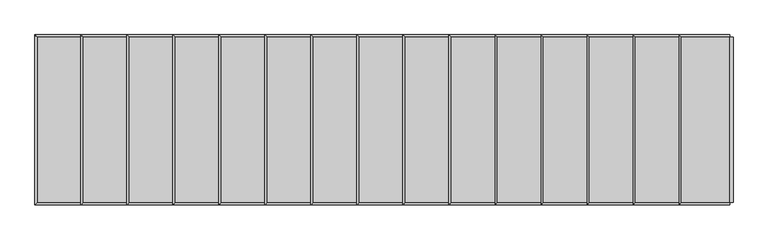
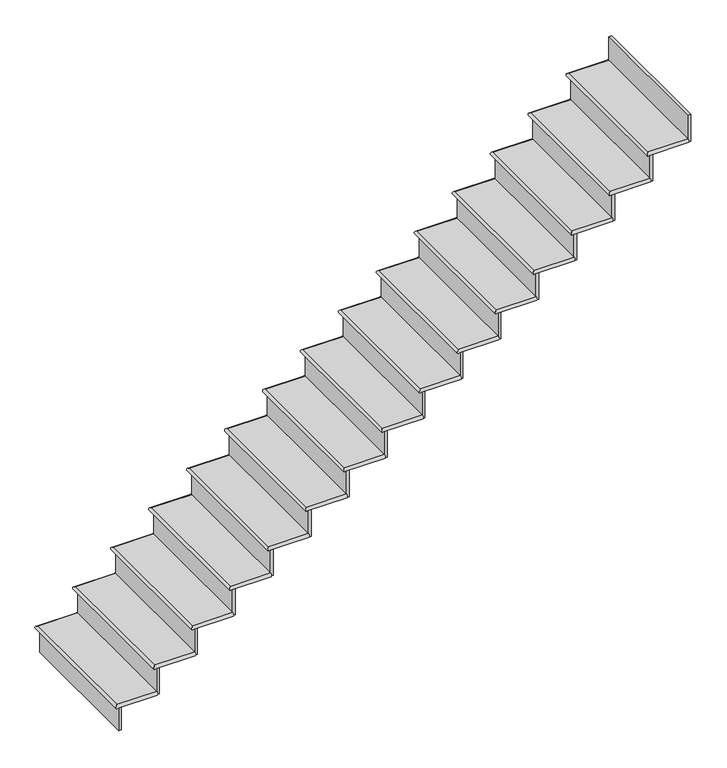
"""IFC4 building model written with IfcOpenShell, lengths in millimetres: stair flight geometry."""

import ifcopenshell
import ifcopenshell.guid

model = None  # the IFC model being written
_history = None  # IfcOwnerHistory: only IFC2X3 demands one
_inside = {}  # id of a spatial element -> (the spatial element, [elements in it])
_under = {}  # id of a project, library or spatial element -> (it, [spatial elements below it])
_declared = {}  # id of a project -> (the project, [libraries it declares])
_typed = {}  # id of a type object -> (the type object, [elements of that type])
_made_of = {}  # id of a material, layer set ... -> (it, [elements and type objects made of it])


def new_model(schema):
    """Start an empty IFC model of exactly this schema.

    Asked for "IFC4X3", IfcOpenShell would pick the latest addendum, in which some entities
    have other attributes; the version numbers below select the first issue.
    IFC2X3 requires an IfcOwnerHistory on every rooted entity: one is made here for all.
    """
    global model, _history
    if schema == "IFC4X3":
        model = ifcopenshell.file(schema_version=(4, 3, 0, 0))
    else:
        model = ifcopenshell.file(schema=schema)
    _inside.clear()
    _under.clear()
    _declared.clear()
    _typed.clear()
    _made_of.clear()
    _history = None
    if model.schema == "IFC2X3":
        org = make("IfcOrganization", Name="unknown")
        user = make(
            "IfcPersonAndOrganization",
            ThePerson=make("IfcPerson", FamilyName="unknown"),
            TheOrganization=org,
        )
        app = make(
            "IfcApplication",
            ApplicationDeveloper=org,
            Version="unknown",
            ApplicationFullName="unknown",
            ApplicationIdentifier="unknown",
        )
        _history = make(
            "IfcOwnerHistory",
            OwningUser=user,
            OwningApplication=app,
            ChangeAction="ADDED",
            CreationDate=0,
        )
    return model


def make(cls, **values):
    """One entity of the class cls with the attributes given. An attribute that is None is left unset."""
    return model.create_entity(
        cls, **{name: value for name, value in values.items() if value is not None}
    )


def rooted(cls, **values):
    """An entity with a GlobalId (a new one), such as an element, a storey or a relation."""
    return make(cls, GlobalId=ifcopenshell.guid.new(), OwnerHistory=_history, **values)


def si_unit(unit_type, name, prefix=None):
    """IfcSIUnit, for example si_unit("LENGTHUNIT", "METRE", prefix="MILLI")."""
    return make("IfcSIUnit", UnitType=unit_type, Prefix=prefix, Name=name)


def assignment(units):
    """IfcUnitAssignment: the units of a project."""
    return None if units is None else make("IfcUnitAssignment", Units=units)


def point(xyz):
    """IfcCartesianPoint."""
    return None if xyz is None else make("IfcCartesianPoint", Coordinates=xyz)


def direction(xyz):
    """IfcDirection."""
    return None if xyz is None else make("IfcDirection", DirectionRatios=xyz)


def frame(location, z_axis=None, x_axis=None):
    """IfcAxis2Placement3D, a coordinate frame: its origin and axes. An axis left out is left unset."""
    return make(
        "IfcAxis2Placement3D",
        Location=point(location),
        Axis=direction(z_axis),
        RefDirection=direction(x_axis),
    )


def origin():
    """The frame at (0, 0, 0) with its axes left unset."""
    return frame((0.0, 0.0, 0.0))


def place(relative_to, where):
    """IfcLocalPlacement: puts the frame where relative to a parent placement (None: the world)."""
    return make(
        "IfcLocalPlacement", PlacementRelTo=relative_to, RelativePlacement=where
    )


def context(
    kind, dimensions, precision=None, world=None, true_north=None, identifier=None
):
    """IfcGeometricRepresentationContext, for example the 3D "Model" context."""
    return make(
        "IfcGeometricRepresentationContext",
        ContextIdentifier=identifier,
        ContextType=kind,
        CoordinateSpaceDimension=dimensions,
        Precision=precision,
        WorldCoordinateSystem=world,
        TrueNorth=true_north,
    )


def project(units=None, contexts=None):
    """IfcProject with its units and contexts."""
    return rooted(
        "IfcProject",
        Name="project",
        RepresentationContexts=contexts,
        UnitsInContext=assignment(units),
    )


def spatial(cls, under=None, at=None, **own):
    """A site, building, storey or space (cls), placed at a placement, below another one or the project."""
    s = rooted(cls, ObjectPlacement=at, **own)
    if under is not None:
        _under.setdefault(under.id(), (under, []))[1].append(s)
    return s


def circle_curve(where, radius):
    """IfcCircle in the frame where."""
    return make("IfcCircle", Position=where, Radius=radius)


def ellipse_curve(where, semi_axis1, semi_axis2):
    """IfcEllipse in the frame where."""
    return make(
        "IfcEllipse", Position=where, SemiAxis1=semi_axis1, SemiAxis2=semi_axis2
    )


def faces_of(points, faces, orient=None, outer=None):
    """IfcFace entities. A face is a list of loops; a loop is a list of indices into points, from 0.

    orient and outer hold one flag for each loop. By default every Orientation is true, the
    first loop of a face is its IfcFaceOuterBound and the others are IfcFaceBound.
    """
    made = []
    for i, loops in enumerate(faces):
        bounds = []
        for j, loop in enumerate(loops):
            is_outer = j == 0 if outer is None else outer[i][j]
            bounds.append(
                make(
                    "IfcFaceOuterBound" if is_outer else "IfcFaceBound",
                    Bound=make("IfcPolyLoop", Polygon=[points[k] for k in loop]),
                    Orientation=True if orient is None else orient[i][j],
                )
            )
        made.append(make("IfcFace", Bounds=bounds))
    return made


def faceted_brep(points, faces, orient=None, outer=None, voids=None):
    """IfcFacetedBrep: a solid bounded by flat faces; with voids (closed shells), ...WithVoids."""
    shared = [point(p) for p in points]
    hull = make("IfcClosedShell", CfsFaces=faces_of(shared, faces, orient, outer))
    if voids is None:
        return make("IfcFacetedBrep", Outer=hull)
    return make(
        "IfcFacetedBrepWithVoids",
        Outer=hull,
        Voids=[
            make(cls, CfsFaces=faces_of(shared, fs, o, b)) for cls, fs, o, b in voids
        ],
    )


def shape(context_of_items, identifier, shape_type, items):
    """IfcShapeRepresentation: the items that make up one representation, for example the "Body"."""
    return make(
        "IfcShapeRepresentation",
        ContextOfItems=context_of_items,
        RepresentationIdentifier=identifier,
        RepresentationType=shape_type,
        Items=items,
    )


def source(mapping_origin, context_of_items, identifier, shape_type, items):
    """IfcRepresentationMap: a shape defined once, which mapped items show again and again."""
    return make(
        "IfcRepresentationMap",
        MappingOrigin=mapping_origin,
        MappedRepresentation=shape(context_of_items, identifier, shape_type, items),
    )


def transform(
    local_origin,
    x_axis=None,
    y_axis=None,
    z_axis=None,
    scale=None,
    scale2=None,
    scale3=None,
    uniform=True,
):
    """IfcCartesianTransformationOperator3D, or its non-uniform kind. x_axis, y_axis, z_axis: its Axis1, 2, 3."""
    if uniform:
        return make(
            "IfcCartesianTransformationOperator3D",
            Axis1=direction(x_axis),
            Axis2=direction(y_axis),
            LocalOrigin=point(local_origin),
            Scale=scale,
            Axis3=direction(z_axis),
        )
    return make(
        "IfcCartesianTransformationOperator3DnonUniform",
        Axis1=direction(x_axis),
        Axis2=direction(y_axis),
        LocalOrigin=point(local_origin),
        Scale=scale,
        Axis3=direction(z_axis),
        Scale2=scale2,
        Scale3=scale3,
    )


def mapped(mapping_source, mapping_target):
    """IfcMappedItem: shows the shape of a source again, moved by a transform."""
    return make(
        "IfcMappedItem", MappingSource=mapping_source, MappingTarget=mapping_target
    )


def made_of(thing, what):
    """Note that an element or type object is made of a material, layer set ...; save() writes the relation."""
    if what is not None:
        _made_of.setdefault(what.id(), (what, []))[1].append(thing)
    return thing


def element(
    cls,
    number,
    at=None,
    inside=None,
    cuts=None,
    type_object=None,
    material=None,
    context=None,
    identifier="Body",
    shape_type=None,
    held_by="IfcProductDefinitionShape",
    body=None,
    shapes=None,
    **own,
):
    """One element of the class cls, such as IfcWall. Its Tag is "e" and its number.

    at: its placement. inside: the storey or other place that contains it. cuts: it is an
    opening in that element (IfcRelVoidsElement). A single representation is given by context,
    identifier, shape_type and body (its items); several are given by shapes. held_by: the class
    of the entity that holds the representations. save() writes the other relations.
    """
    e = rooted(cls, Tag="e%d" % number, ObjectPlacement=at, **own)
    if body is not None:
        shapes = [shape(context, identifier, shape_type, body)]
    if shapes is not None:
        e.Representation = make(held_by, Representations=shapes)
    if inside is not None:
        _inside.setdefault(inside.id(), (inside, []))[1].append(e)
    if cuts is not None:
        rooted(
            "IfcRelVoidsElement", RelatingBuildingElement=cuts, RelatedOpeningElement=e
        )
    if type_object is not None:
        _typed.setdefault(type_object.id(), (type_object, []))[1].append(e)
    return made_of(e, material)


def aggregate(whole, parts):
    """IfcRelAggregates: a whole, such as a stair, and the parts it consists of."""
    return rooted("IfcRelAggregates", RelatingObject=whole, RelatedObjects=parts)


def save(model, path):
    """Write the relations noted so far, then the file.

    IfcRelAggregates (storeys below a building ...), IfcRelContainedInSpatialStructure (elements
    in a storey), IfcRelDefinesByType, IfcRelAssociatesMaterial and IfcRelDeclares: one each for
    every whole, place, type object, material and project.
    """
    for whole, parts in _under.values():
        aggregate(whole, parts)
    for where, things in _inside.values():
        rooted(
            "IfcRelContainedInSpatialStructure",
            RelatedElements=things,
            RelatingStructure=where,
        )
    for kind, things in _typed.values():
        rooted("IfcRelDefinesByType", RelatedObjects=things, RelatingType=kind)
    for what, things in _made_of.values():
        rooted("IfcRelAssociatesMaterial", RelatedObjects=things, RelatingMaterial=what)
    for by, libraries in _declared.values():
        rooted("IfcRelDeclares", RelatingContext=by, RelatedDefinitions=libraries)
    model.write(path)


def plane_surface(at):
    """IfcPlane: the flat surface through the origin of the frame at, square to its z axis."""
    return make("IfcPlane", Position=at)


def cylinder_surface(at, radius):
    """IfcCylindricalSurface: all points at the distance radius from the z axis of the frame at."""
    return make("IfcCylindricalSurface", Position=at, Radius=radius)


def advanced_brep(points, edges, surfaces, faces):
    """IfcAdvancedBrep: a solid bounded by faces that lie on surfaces and meet in shared edges.

    An edge is (start, end): straight between two places in points (the first is 0);
    or (start, end, curve); or (start, end, curve, False) where it runs against its curve.
    A face is (place in surfaces, loops), or (place, loops, False) where it looks against
    its surface's normal. A loop lists edges by number (the first is 1), with a minus sign
    where the edge is run from its end to its start. The first loop is the outer one.
    """
    corners = [point(p) for p in points]
    vertices = [make("IfcVertexPoint", VertexGeometry=c) for c in corners]
    made = []
    for start, end, *more in edges:
        made.append(
            make(
                "IfcEdgeCurve",
                EdgeStart=vertices[start],
                EdgeEnd=vertices[end],
                EdgeGeometry=more[0] if more else make("IfcPolyline", Points=[corners[start], corners[end]]),
                SameSense=more[1] if len(more) > 1 else True,
            )
        )
    hull = []
    for where, loops, *sense in faces:
        bounds = []
        for j, loop in enumerate(loops):
            ring = [make("IfcOrientedEdge", EdgeElement=made[abs(k) - 1], Orientation=k > 0) for k in loop]
            bounds.append(
                make(
                    "IfcFaceOuterBound" if j == 0 else "IfcFaceBound",
                    Bound=make("IfcEdgeLoop", EdgeList=ring),
                    Orientation=True,
                )
            )
        hull.append(make("IfcAdvancedFace", Bounds=bounds, FaceSurface=surfaces[where], SameSense=sense[0] if sense else True))
    return make("IfcAdvancedBrep", Outer=make("IfcClosedShell", CfsFaces=hull))


def stair_flight_3790ce72(model_context):
    return source(origin(), model_context, "Body", "SolidModel", [
        advanced_brep(
        [(-27218.1481446, 3955.9128094, 165.1), (-27218.1481446, 3955.9128094, 190.5), (-27218.1481446, 4870.3128094, 190.5), (-27218.1481446, 4870.3128094, 165.1), (-26951.4481446, 3955.9128094, 190.5), (-26951.4481446, 4870.3128094, 190.5), (-26951.4481446, 4870.3128094, 165.1), (-26951.4481446, 3955.9128094, 165.1)],
        [
            (0, 1, ellipse_curve(frame((-27218.1481446, 3955.9128094, 177.8), z_axis=(-0.7071067811865447, 0.7071067811865502, 0.0), x_axis=(-0.7071067811865501, -0.7071067811865449, 0.0)), 17.9605122, 12.7)),
            (1, 2),
            (2, 3, ellipse_curve(frame((-27218.1481446, 4870.3128094, 177.8), z_axis=(-0.7071067811865502, -0.7071067811865448, 0.0), x_axis=(0.7071067811865448, -0.7071067811865502, 0.0)), 17.9605122, 12.7)),
            (3, 0),
            (4, 5),
            (5, 2),
            (1, 4),
            (6, 7),
            (7, 0),
            (3, 6),
            (4, 7, circle_curve(frame((-26951.4481446, 3955.9128094, 177.8), z_axis=(1.0, 0.0, 0.0), x_axis=(0.0, 1.0, 0.0)), 12.7)),
            (6, 5, circle_curve(frame((-26951.4481446, 4870.3128094, 177.8), z_axis=(1.0, 0.0, 0.0), x_axis=(0.0, -1.0, 0.0)), 12.7)),
        ],
        [
            cylinder_surface(frame((-27218.1481446, 3955.9128094, 177.8), z_axis=(0.0, -1.0, 0.0), x_axis=(1.0, 0.0, 0.0)), 12.7),
            plane_surface(frame((-27230.8481446, 4870.3128094, 190.5), z_axis=(0.0, 0.0, 1.0), x_axis=(-1.0, 0.0, 0.0))),
            plane_surface(frame((-27230.8481446, 4870.3128094, 165.1), z_axis=(0.0, 0.0, -1.0), x_axis=(1.0, 0.0, 0.0))),
            plane_surface(frame((-26951.4481446, 3955.9128094, 190.5), z_axis=(1.0, 0.0, 0.0), x_axis=(0.0, 0.0, -1.0))),
            cylinder_surface(frame((-26951.4481446, 3955.9128094, 177.8), z_axis=(1.0, 0.0, 0.0), x_axis=(0.0, 1.0, 0.0)), 12.7),
            cylinder_surface(frame((-27218.1481446, 4870.3128094, 177.8), z_axis=(-1.0, 0.0, 0.0), x_axis=(0.0, -1.0, 0.0)), 12.7),
        ],
        [
            (0, [[1, 2, 3, 4]]),
            (1, [[5, 6, -2, 7]]),
            (2, [[8, 9, -4, 10]]),
            (3, [[-5, 11, -8, 12]]),
            (4, [[-11, -7, -1, -9]]),
            (5, [[-3, -6, -12, -10]]),
        ],
    ),
        faceted_brep([(-27205.4481446, 3955.9128094, 165.1), (-27205.4481446, 3955.9128094, 0.0), (-27186.3981446, 3955.9128094, 0.0), (-27186.3981446, 3955.9128094, 165.1), (-27205.4481446, 4870.3128094, 165.1), (-27186.3981446, 4870.3128094, 165.1), (-27186.3981446, 4870.3128094, 0.0), (-27205.4481446, 4870.3128094, 0.0)], [[[0, 1, 2, 3]], [[4, 5, 6, 7]], [[1, 0, 4, 7]], [[2, 1, 7, 6]], [[3, 2, 6, 5]], [[0, 3, 5, 4]]]),
        faceted_brep([(-26951.4481446, 3955.9128094, 355.6), (-26951.4481446, 3955.9128094, 165.1), (-26932.3981446, 3955.9128094, 165.1), (-26932.3981446, 3955.9128094, 355.6), (-26951.4481446, 4870.3128094, 355.6), (-26932.3981446, 4870.3128094, 355.6), (-26932.3981446, 4870.3128094, 165.1), (-26951.4481446, 4870.3128094, 165.1)], [[[0, 1, 2, 3]], [[4, 5, 6, 7]], [[1, 0, 4, 7]], [[2, 1, 7, 6]], [[3, 2, 6, 5]], [[0, 3, 5, 4]]]),
        advanced_brep(
        [(-26697.4481446, 3955.9128094, 381.0), (-26697.4481446, 4870.3128094, 381.0), (-26964.1481446, 4870.3128094, 381.0), (-26964.1481446, 3955.9128094, 381.0), (-26697.4481446, 4870.3128094, 355.6), (-26697.4481446, 3955.9128094, 355.6), (-26964.1481446, 3955.9128094, 355.6), (-26964.1481446, 4870.3128094, 355.6)],
        [
            (0, 1),
            (1, 2),
            (2, 3),
            (3, 0),
            (4, 5),
            (5, 6),
            (6, 7),
            (7, 4),
            (0, 5, circle_curve(frame((-26697.4481446, 3955.9128094, 368.3), z_axis=(1.0, 0.0, 0.0), x_axis=(0.0, 1.0, 0.0)), 12.7)),
            (4, 1, circle_curve(frame((-26697.4481446, 4870.3128094, 368.3), z_axis=(1.0, 0.0, 0.0), x_axis=(0.0, -1.0, 0.0)), 12.7)),
            (6, 3, ellipse_curve(frame((-26964.1481446, 3955.9128094, 368.3), z_axis=(-0.7071067811865456, 0.7071067811865496, 0.0), x_axis=(-0.7071067811865496, -0.7071067811865455, 0.0)), 17.9605122, 12.7)),
            (2, 7, ellipse_curve(frame((-26964.1481446, 4870.3128094, 368.3), z_axis=(-0.7071067811865496, -0.7071067811865455, 0.0), x_axis=(0.7071067811865456, -0.7071067811865496, 0.0)), 17.9605122, 12.7)),
        ],
        [
            plane_surface(frame((-27230.8481446, 4870.3128094, 381.0), z_axis=(0.0, 0.0, 1.0), x_axis=(-1.0, 0.0, 0.0))),
            plane_surface(frame((-27230.8481446, 4870.3128094, 355.6), z_axis=(0.0, 0.0, -1.0), x_axis=(1.0, 0.0, 0.0))),
            plane_surface(frame((-26697.4481446, 3955.9128094, 381.0), z_axis=(1.0, 0.0, 0.0), x_axis=(0.0, 0.0, -1.0))),
            cylinder_surface(frame((-26964.1481446, 3955.9128094, 368.3), z_axis=(0.0, -1.0, 0.0), x_axis=(1.0, 0.0, 0.0)), 12.7),
            cylinder_surface(frame((-26697.4481446, 3955.9128094, 368.3), z_axis=(1.0, 0.0, 0.0), x_axis=(0.0, 1.0, 0.0)), 12.7),
            cylinder_surface(frame((-26964.1481446, 4870.3128094, 368.3), z_axis=(-1.0, 0.0, 0.0), x_axis=(0.0, -1.0, 0.0)), 12.7),
        ],
        [
            (0, [[1, 2, 3, 4]]),
            (1, [[5, 6, 7, 8]]),
            (2, [[-1, 9, -5, 10]]),
            (3, [[11, -3, 12, -7]]),
            (4, [[-9, -4, -11, -6]]),
            (5, [[-12, -2, -10, -8]]),
        ],
    ),
        faceted_brep([(-26697.4481446, 3955.9128094, 546.1), (-26697.4481446, 3955.9128094, 355.6), (-26678.3981446, 3955.9128094, 355.6), (-26678.3981446, 3955.9128094, 546.1), (-26697.4481446, 4870.3128094, 546.1), (-26678.3981446, 4870.3128094, 546.1), (-26678.3981446, 4870.3128094, 355.6), (-26697.4481446, 4870.3128094, 355.6)], [[[0, 1, 2, 3]], [[4, 5, 6, 7]], [[1, 0, 4, 7]], [[2, 1, 7, 6]], [[3, 2, 6, 5]], [[0, 3, 5, 4]]]),
        advanced_brep(
        [(-26443.4481446, 3955.9128094, 571.5), (-26443.4481446, 4870.3128094, 571.5), (-26710.1481446, 4870.3128094, 571.5), (-26710.1481446, 3955.9128094, 571.5), (-26443.4481446, 4870.3128094, 546.1), (-26443.4481446, 3955.9128094, 546.1), (-26710.1481446, 3955.9128094, 546.1), (-26710.1481446, 4870.3128094, 546.1)],
        [
            (0, 1),
            (1, 2),
            (2, 3),
            (3, 0),
            (4, 5),
            (5, 6),
            (6, 7),
            (7, 4),
            (0, 5, circle_curve(frame((-26443.4481446, 3955.9128094, 558.8), z_axis=(1.0, 0.0, 0.0), x_axis=(0.0, 1.0, 0.0)), 12.7)),
            (4, 1, circle_curve(frame((-26443.4481446, 4870.3128094, 558.8), z_axis=(1.0, 0.0, 0.0), x_axis=(0.0, -1.0, 0.0)), 12.7)),
            (6, 3, ellipse_curve(frame((-26710.1481446, 3955.9128094, 558.8), z_axis=(-0.7071067811865456, 0.7071067811865496, 0.0), x_axis=(-0.7071067811865496, -0.7071067811865455, 0.0)), 17.9605122, 12.7)),
            (2, 7, ellipse_curve(frame((-26710.1481446, 4870.3128094, 558.8), z_axis=(-0.7071067811865496, -0.7071067811865455, 0.0), x_axis=(0.7071067811865456, -0.7071067811865496, 0.0)), 17.9605122, 12.7)),
        ],
        [
            plane_surface(frame((-26976.8481446, 4870.3128094, 571.5), z_axis=(0.0, 0.0, 1.0), x_axis=(-1.0, 0.0, 0.0))),
            plane_surface(frame((-26976.8481446, 4870.3128094, 546.1), z_axis=(0.0, 0.0, -1.0), x_axis=(1.0, 0.0, 0.0))),
            plane_surface(frame((-26443.4481446, 3955.9128094, 571.5), z_axis=(1.0, 0.0, 0.0), x_axis=(0.0, 0.0, -1.0))),
            cylinder_surface(frame((-26710.1481446, 3955.9128094, 558.8), z_axis=(0.0, -1.0, 0.0), x_axis=(1.0, 0.0, 0.0)), 12.7),
            cylinder_surface(frame((-26443.4481446, 3955.9128094, 558.8), z_axis=(1.0, 0.0, 0.0), x_axis=(0.0, 1.0, 0.0)), 12.7),
            cylinder_surface(frame((-26710.1481446, 4870.3128094, 558.8), z_axis=(-1.0, 0.0, 0.0), x_axis=(0.0, -1.0, 0.0)), 12.7),
        ],
        [
            (0, [[1, 2, 3, 4]]),
            (1, [[5, 6, 7, 8]]),
            (2, [[-1, 9, -5, 10]]),
            (3, [[11, -3, 12, -7]]),
            (4, [[-9, -4, -11, -6]]),
            (5, [[-12, -2, -10, -8]]),
        ],
    ),
        faceted_brep([(-26443.4481446, 3955.9128094, 736.6), (-26443.4481446, 3955.9128094, 546.1), (-26424.3981446, 3955.9128094, 546.1), (-26424.3981446, 3955.9128094, 736.6), (-26443.4481446, 4870.3128094, 736.6), (-26424.3981446, 4870.3128094, 736.6), (-26424.3981446, 4870.3128094, 546.1), (-26443.4481446, 4870.3128094, 546.1)], [[[0, 1, 2, 3]], [[4, 5, 6, 7]], [[1, 0, 4, 7]], [[2, 1, 7, 6]], [[3, 2, 6, 5]], [[0, 3, 5, 4]]]),
        advanced_brep(
        [(-26189.4481446, 3955.9128094, 762.0), (-26189.4481446, 4870.3128094, 762.0), (-26456.1481446, 4870.3128094, 762.0), (-26456.1481446, 3955.9128094, 762.0), (-26189.4481446, 4870.3128094, 736.6), (-26189.4481446, 3955.9128094, 736.6), (-26456.1481446, 3955.9128094, 736.6), (-26456.1481446, 4870.3128094, 736.6)],
        [
            (0, 1),
            (1, 2),
            (2, 3),
            (3, 0),
            (4, 5),
            (5, 6),
            (6, 7),
            (7, 4),
            (0, 5, circle_curve(frame((-26189.4481446, 3955.9128094, 749.3), z_axis=(1.0, 0.0, 0.0), x_axis=(0.0, 1.0, 0.0)), 12.7)),
            (4, 1, circle_curve(frame((-26189.4481446, 4870.3128094, 749.3), z_axis=(1.0, 0.0, 0.0), x_axis=(0.0, -1.0, 0.0)), 12.7)),
            (6, 3, ellipse_curve(frame((-26456.1481446, 3955.9128094, 749.3), z_axis=(-0.7071067811865456, 0.7071067811865496, 0.0), x_axis=(-0.7071067811865496, -0.7071067811865455, 0.0)), 17.9605122, 12.7)),
            (2, 7, ellipse_curve(frame((-26456.1481446, 4870.3128094, 749.3), z_axis=(-0.7071067811865496, -0.7071067811865455, 0.0), x_axis=(0.7071067811865456, -0.7071067811865496, 0.0)), 17.9605122, 12.7)),
        ],
        [
            plane_surface(frame((-26722.8481446, 4870.3128094, 762.0), z_axis=(0.0, 0.0, 1.0), x_axis=(-1.0, 0.0, 0.0))),
            plane_surface(frame((-26722.8481446, 4870.3128094, 736.6), z_axis=(0.0, 0.0, -1.0), x_axis=(1.0, 0.0, 0.0))),
            plane_surface(frame((-26189.4481446, 3955.9128094, 762.0), z_axis=(1.0, 0.0, 0.0), x_axis=(0.0, 0.0, -1.0))),
            cylinder_surface(frame((-26456.1481446, 3955.9128094, 749.3), z_axis=(0.0, -1.0, 0.0), x_axis=(1.0, 0.0, 0.0)), 12.7),
            cylinder_surface(frame((-26189.4481446, 3955.9128094, 749.3), z_axis=(1.0, 0.0, 0.0), x_axis=(0.0, 1.0, 0.0)), 12.7),
            cylinder_surface(frame((-26456.1481446, 4870.3128094, 749.3), z_axis=(-1.0, 0.0, 0.0), x_axis=(0.0, -1.0, 0.0)), 12.7),
        ],
        [
            (0, [[1, 2, 3, 4]]),
            (1, [[5, 6, 7, 8]]),
            (2, [[-1, 9, -5, 10]]),
            (3, [[11, -3, 12, -7]]),
            (4, [[-9, -4, -11, -6]]),
            (5, [[-12, -2, -10, -8]]),
        ],
    ),
        faceted_brep([(-26189.4481446, 3955.9128094, 927.1), (-26189.4481446, 3955.9128094, 736.6), (-26170.3981446, 3955.9128094, 736.6), (-26170.3981446, 3955.9128094, 927.1), (-26189.4481446, 4870.3128094, 927.1), (-26170.3981446, 4870.3128094, 927.1), (-26170.3981446, 4870.3128094, 736.6), (-26189.4481446, 4870.3128094, 736.6)], [[[0, 1, 2, 3]], [[4, 5, 6, 7]], [[1, 0, 4, 7]], [[2, 1, 7, 6]], [[3, 2, 6, 5]], [[0, 3, 5, 4]]]),
        advanced_brep(
        [(-25935.4481446, 3955.9128094, 952.5), (-25935.4481446, 4870.3128094, 952.5), (-26202.1481446, 4870.3128094, 952.5), (-26202.1481446, 3955.9128094, 952.5), (-25935.4481446, 4870.3128094, 927.1), (-25935.4481446, 3955.9128094, 927.1), (-26202.1481446, 3955.9128094, 927.1), (-26202.1481446, 4870.3128094, 927.1)],
        [
            (0, 1),
            (1, 2),
            (2, 3),
            (3, 0),
            (4, 5),
            (5, 6),
            (6, 7),
            (7, 4),
            (0, 5, circle_curve(frame((-25935.4481446, 3955.9128094, 939.8), z_axis=(1.0, 0.0, 0.0), x_axis=(0.0, 1.0, 0.0)), 12.7)),
            (4, 1, circle_curve(frame((-25935.4481446, 4870.3128094, 939.8), z_axis=(1.0, 0.0, 0.0), x_axis=(0.0, -1.0, 0.0)), 12.7)),
            (6, 3, ellipse_curve(frame((-26202.1481446, 3955.9128094, 939.8), z_axis=(-0.7071067811865456, 0.7071067811865496, 0.0), x_axis=(-0.7071067811865496, -0.7071067811865455, 0.0)), 17.9605122, 12.7)),
            (2, 7, ellipse_curve(frame((-26202.1481446, 4870.3128094, 939.8), z_axis=(-0.7071067811865496, -0.7071067811865455, 0.0), x_axis=(0.7071067811865456, -0.7071067811865496, 0.0)), 17.9605122, 12.7)),
        ],
        [
            plane_surface(frame((-26468.8481446, 4870.3128094, 952.5), z_axis=(0.0, 0.0, 1.0), x_axis=(-1.0, 0.0, 0.0))),
            plane_surface(frame((-26468.8481446, 4870.3128094, 927.1), z_axis=(0.0, 0.0, -1.0), x_axis=(1.0, 0.0, 0.0))),
            plane_surface(frame((-25935.4481446, 3955.9128094, 952.5), z_axis=(1.0, 0.0, 0.0), x_axis=(0.0, 0.0, -1.0))),
            cylinder_surface(frame((-26202.1481446, 3955.9128094, 939.8), z_axis=(0.0, -1.0, 0.0), x_axis=(1.0, 0.0, 0.0)), 12.7),
            cylinder_surface(frame((-25935.4481446, 3955.9128094, 939.8), z_axis=(1.0, 0.0, 0.0), x_axis=(0.0, 1.0, 0.0)), 12.7),
            cylinder_surface(frame((-26202.1481446, 4870.3128094, 939.8), z_axis=(-1.0, 0.0, 0.0), x_axis=(0.0, -1.0, 0.0)), 12.7),
        ],
        [
            (0, [[1, 2, 3, 4]]),
            (1, [[5, 6, 7, 8]]),
            (2, [[-1, 9, -5, 10]]),
            (3, [[11, -3, 12, -7]]),
            (4, [[-9, -4, -11, -6]]),
            (5, [[-12, -2, -10, -8]]),
        ],
    ),
        faceted_brep([(-25935.4481446, 3955.9128094, 1117.6), (-25935.4481446, 3955.9128094, 927.1), (-25916.3981446, 3955.9128094, 927.1), (-25916.3981446, 3955.9128094, 1117.6), (-25935.4481446, 4870.3128094, 1117.6), (-25916.3981446, 4870.3128094, 1117.6), (-25916.3981446, 4870.3128094, 927.1), (-25935.4481446, 4870.3128094, 927.1)], [[[0, 1, 2, 3]], [[4, 5, 6, 7]], [[1, 0, 4, 7]], [[2, 1, 7, 6]], [[3, 2, 6, 5]], [[0, 3, 5, 4]]]),
        advanced_brep(
        [(-25681.4481446, 3955.9128094, 1143.0), (-25681.4481446, 4870.3128094, 1143.0), (-25948.1481446, 4870.3128094, 1143.0), (-25948.1481446, 3955.9128094, 1143.0), (-25681.4481446, 4870.3128094, 1117.6), (-25681.4481446, 3955.9128094, 1117.6), (-25948.1481446, 3955.9128094, 1117.6), (-25948.1481446, 4870.3128094, 1117.6)],
        [
            (0, 1),
            (1, 2),
            (2, 3),
            (3, 0),
            (4, 5),
            (5, 6),
            (6, 7),
            (7, 4),
            (0, 5, circle_curve(frame((-25681.4481446, 3955.9128094, 1130.3), z_axis=(1.0, 0.0, 0.0), x_axis=(0.0, 1.0, 0.0)), 12.7)),
            (4, 1, circle_curve(frame((-25681.4481446, 4870.3128094, 1130.3), z_axis=(1.0, 0.0, 0.0), x_axis=(0.0, -1.0, 0.0)), 12.7)),
            (6, 3, ellipse_curve(frame((-25948.1481446, 3955.9128094, 1130.3), z_axis=(-0.7071067811865456, 0.7071067811865496, 0.0), x_axis=(-0.7071067811865496, -0.7071067811865455, 0.0)), 17.9605122, 12.7)),
            (2, 7, ellipse_curve(frame((-25948.1481446, 4870.3128094, 1130.3), z_axis=(-0.7071067811865496, -0.7071067811865455, 0.0), x_axis=(0.7071067811865456, -0.7071067811865496, 0.0)), 17.9605122, 12.7)),
        ],
        [
            plane_surface(frame((-26214.8481446, 4870.3128094, 1143.0), z_axis=(0.0, 0.0, 1.0), x_axis=(-1.0, 0.0, 0.0))),
            plane_surface(frame((-26214.8481446, 4870.3128094, 1117.6), z_axis=(0.0, 0.0, -1.0), x_axis=(1.0, 0.0, 0.0))),
            plane_surface(frame((-25681.4481446, 3955.9128094, 1143.0), z_axis=(1.0, 0.0, 0.0), x_axis=(0.0, 0.0, -1.0))),
            cylinder_surface(frame((-25948.1481446, 3955.9128094, 1130.3), z_axis=(0.0, -1.0, 0.0), x_axis=(1.0, 0.0, 0.0)), 12.7),
            cylinder_surface(frame((-25681.4481446, 3955.9128094, 1130.3), z_axis=(1.0, 0.0, 0.0), x_axis=(0.0, 1.0, 0.0)), 12.7),
            cylinder_surface(frame((-25948.1481446, 4870.3128094, 1130.3), z_axis=(-1.0, 0.0, 0.0), x_axis=(0.0, -1.0, 0.0)), 12.7),
        ],
        [
            (0, [[1, 2, 3, 4]]),
            (1, [[5, 6, 7, 8]]),
            (2, [[-1, 9, -5, 10]]),
            (3, [[11, -3, 12, -7]]),
            (4, [[-9, -4, -11, -6]]),
            (5, [[-12, -2, -10, -8]]),
        ],
    ),
        faceted_brep([(-25681.4481446, 3955.9128094, 1308.1), (-25681.4481446, 3955.9128094, 1117.6), (-25662.3981446, 3955.9128094, 1117.6), (-25662.3981446, 3955.9128094, 1308.1), (-25681.4481446, 4870.3128094, 1308.1), (-25662.3981446, 4870.3128094, 1308.1), (-25662.3981446, 4870.3128094, 1117.6), (-25681.4481446, 4870.3128094, 1117.6)], [[[0, 1, 2, 3]], [[4, 5, 6, 7]], [[1, 0, 4, 7]], [[2, 1, 7, 6]], [[3, 2, 6, 5]], [[0, 3, 5, 4]]]),
        advanced_brep(
        [(-25427.4481446, 3955.9128094, 1333.5), (-25427.4481446, 4870.3128094, 1333.5), (-25694.1481446, 4870.3128094, 1333.5), (-25694.1481446, 3955.9128094, 1333.5), (-25427.4481446, 4870.3128094, 1308.1), (-25427.4481446, 3955.9128094, 1308.1), (-25694.1481446, 3955.9128094, 1308.1), (-25694.1481446, 4870.3128094, 1308.1)],
        [
            (0, 1),
            (1, 2),
            (2, 3),
            (3, 0),
            (4, 5),
            (5, 6),
            (6, 7),
            (7, 4),
            (0, 5, circle_curve(frame((-25427.4481446, 3955.9128094, 1320.8), z_axis=(1.0, 0.0, 0.0), x_axis=(0.0, 1.0, 0.0)), 12.7)),
            (4, 1, circle_curve(frame((-25427.4481446, 4870.3128094, 1320.8), z_axis=(1.0, 0.0, 0.0), x_axis=(0.0, -1.0, 0.0)), 12.7)),
            (6, 3, ellipse_curve(frame((-25694.1481446, 3955.9128094, 1320.8), z_axis=(-0.7071067811865456, 0.7071067811865496, 0.0), x_axis=(-0.7071067811865496, -0.7071067811865455, 0.0)), 17.9605122, 12.7)),
            (2, 7, ellipse_curve(frame((-25694.1481446, 4870.3128094, 1320.8), z_axis=(-0.7071067811865496, -0.7071067811865455, 0.0), x_axis=(0.7071067811865456, -0.7071067811865496, 0.0)), 17.9605122, 12.7)),
        ],
        [
            plane_surface(frame((-25960.8481446, 4870.3128094, 1333.5), z_axis=(0.0, 0.0, 1.0), x_axis=(-1.0, 0.0, 0.0))),
            plane_surface(frame((-25960.8481446, 4870.3128094, 1308.1), z_axis=(0.0, 0.0, -1.0), x_axis=(1.0, 0.0, 0.0))),
            plane_surface(frame((-25427.4481446, 3955.9128094, 1333.5), z_axis=(1.0, 0.0, 0.0), x_axis=(0.0, 0.0, -1.0))),
            cylinder_surface(frame((-25694.1481446, 3955.9128094, 1320.8), z_axis=(0.0, -1.0, 0.0), x_axis=(1.0, 0.0, 0.0)), 12.7),
            cylinder_surface(frame((-25427.4481446, 3955.9128094, 1320.8), z_axis=(1.0, 0.0, 0.0), x_axis=(0.0, 1.0, 0.0)), 12.7),
            cylinder_surface(frame((-25694.1481446, 4870.3128094, 1320.8), z_axis=(-1.0, 0.0, 0.0), x_axis=(0.0, -1.0, 0.0)), 12.7),
        ],
        [
            (0, [[1, 2, 3, 4]]),
            (1, [[5, 6, 7, 8]]),
            (2, [[-1, 9, -5, 10]]),
            (3, [[11, -3, 12, -7]]),
            (4, [[-9, -4, -11, -6]]),
            (5, [[-12, -2, -10, -8]]),
        ],
    ),
        faceted_brep([(-25427.4481446, 3955.9128094, 1498.6), (-25427.4481446, 3955.9128094, 1308.1), (-25408.3981446, 3955.9128094, 1308.1), (-25408.3981446, 3955.9128094, 1498.6), (-25427.4481446, 4870.3128094, 1498.6), (-25408.3981446, 4870.3128094, 1498.6), (-25408.3981446, 4870.3128094, 1308.1), (-25427.4481446, 4870.3128094, 1308.1)], [[[0, 1, 2, 3]], [[4, 5, 6, 7]], [[1, 0, 4, 7]], [[2, 1, 7, 6]], [[3, 2, 6, 5]], [[0, 3, 5, 4]]]),
        advanced_brep(
        [(-25173.4481446, 3955.9128094, 1524.0), (-25173.4481446, 4870.3128094, 1524.0), (-25440.1481446, 4870.3128094, 1524.0), (-25440.1481446, 3955.9128094, 1524.0), (-25173.4481446, 4870.3128094, 1498.6), (-25173.4481446, 3955.9128094, 1498.6), (-25440.1481446, 3955.9128094, 1498.6), (-25440.1481446, 4870.3128094, 1498.6)],
        [
            (0, 1),
            (1, 2),
            (2, 3),
            (3, 0),
            (4, 5),
            (5, 6),
            (6, 7),
            (7, 4),
            (0, 5, circle_curve(frame((-25173.4481446, 3955.9128094, 1511.3), z_axis=(1.0, 0.0, 0.0), x_axis=(0.0, 1.0, 0.0)), 12.7)),
            (4, 1, circle_curve(frame((-25173.4481446, 4870.3128094, 1511.3), z_axis=(1.0, 0.0, 0.0), x_axis=(0.0, -1.0, 0.0)), 12.7)),
            (6, 3, ellipse_curve(frame((-25440.1481446, 3955.9128094, 1511.3), z_axis=(-0.7071067811865456, 0.7071067811865496, 0.0), x_axis=(-0.7071067811865496, -0.7071067811865455, 0.0)), 17.9605122, 12.7)),
            (2, 7, ellipse_curve(frame((-25440.1481446, 4870.3128094, 1511.3), z_axis=(-0.7071067811865496, -0.7071067811865455, 0.0), x_axis=(0.7071067811865456, -0.7071067811865496, 0.0)), 17.9605122, 12.7)),
        ],
        [
            plane_surface(frame((-25706.8481446, 4870.3128094, 1524.0), z_axis=(0.0, 0.0, 1.0), x_axis=(-1.0, 0.0, 0.0))),
            plane_surface(frame((-25706.8481446, 4870.3128094, 1498.6), z_axis=(0.0, 0.0, -1.0), x_axis=(1.0, 0.0, 0.0))),
            plane_surface(frame((-25173.4481446, 3955.9128094, 1524.0), z_axis=(1.0, 0.0, 0.0), x_axis=(0.0, 0.0, -1.0))),
            cylinder_surface(frame((-25440.1481446, 3955.9128094, 1511.3), z_axis=(0.0, -1.0, 0.0), x_axis=(1.0, 0.0, 0.0)), 12.7),
            cylinder_surface(frame((-25173.4481446, 3955.9128094, 1511.3), z_axis=(1.0, 0.0, 0.0), x_axis=(0.0, 1.0, 0.0)), 12.7),
            cylinder_surface(frame((-25440.1481446, 4870.3128094, 1511.3), z_axis=(-1.0, 0.0, 0.0), x_axis=(0.0, -1.0, 0.0)), 12.7),
        ],
        [
            (0, [[1, 2, 3, 4]]),
            (1, [[5, 6, 7, 8]]),
            (2, [[-1, 9, -5, 10]]),
            (3, [[11, -3, 12, -7]]),
            (4, [[-9, -4, -11, -6]]),
            (5, [[-12, -2, -10, -8]]),
        ],
    ),
        faceted_brep([(-25173.4481446, 3955.9128094, 1689.1), (-25173.4481446, 3955.9128094, 1498.6), (-25154.3981446, 3955.9128094, 1498.6), (-25154.3981446, 3955.9128094, 1689.1), (-25173.4481446, 4870.3128094, 1689.1), (-25154.3981446, 4870.3128094, 1689.1), (-25154.3981446, 4870.3128094, 1498.6), (-25173.4481446, 4870.3128094, 1498.6)], [[[0, 1, 2, 3]], [[4, 5, 6, 7]], [[1, 0, 4, 7]], [[2, 1, 7, 6]], [[3, 2, 6, 5]], [[0, 3, 5, 4]]]),
        advanced_brep(
        [(-24919.4481446, 3955.9128094, 1714.5), (-24919.4481446, 4870.3128094, 1714.5), (-25186.1481446, 4870.3128094, 1714.5), (-25186.1481446, 3955.9128094, 1714.5), (-24919.4481446, 4870.3128094, 1689.1), (-24919.4481446, 3955.9128094, 1689.1), (-25186.1481446, 3955.9128094, 1689.1), (-25186.1481446, 4870.3128094, 1689.1)],
        [
            (0, 1),
            (1, 2),
            (2, 3),
            (3, 0),
            (4, 5),
            (5, 6),
            (6, 7),
            (7, 4),
            (0, 5, circle_curve(frame((-24919.4481446, 3955.9128094, 1701.8), z_axis=(1.0, 0.0, 0.0), x_axis=(0.0, 1.0, 0.0)), 12.7)),
            (4, 1, circle_curve(frame((-24919.4481446, 4870.3128094, 1701.8), z_axis=(1.0, 0.0, 0.0), x_axis=(0.0, -1.0, 0.0)), 12.7)),
            (6, 3, ellipse_curve(frame((-25186.1481446, 3955.9128094, 1701.8), z_axis=(-0.7071067811865456, 0.7071067811865496, 0.0), x_axis=(-0.7071067811865496, -0.7071067811865455, 0.0)), 17.9605122, 12.7)),
            (2, 7, ellipse_curve(frame((-25186.1481446, 4870.3128094, 1701.8), z_axis=(-0.7071067811865496, -0.7071067811865455, 0.0), x_axis=(0.7071067811865456, -0.7071067811865496, 0.0)), 17.9605122, 12.7)),
        ],
        [
            plane_surface(frame((-25452.8481446, 4870.3128094, 1714.5), z_axis=(0.0, 0.0, 1.0), x_axis=(-1.0, 0.0, 0.0))),
            plane_surface(frame((-25452.8481446, 4870.3128094, 1689.1), z_axis=(0.0, 0.0, -1.0), x_axis=(1.0, 0.0, 0.0))),
            plane_surface(frame((-24919.4481446, 3955.9128094, 1714.5), z_axis=(1.0, 0.0, 0.0), x_axis=(0.0, 0.0, -1.0))),
            cylinder_surface(frame((-25186.1481446, 3955.9128094, 1701.8), z_axis=(0.0, -1.0, 0.0), x_axis=(1.0, 0.0, 0.0)), 12.7),
            cylinder_surface(frame((-24919.4481446, 3955.9128094, 1701.8), z_axis=(1.0, 0.0, 0.0), x_axis=(0.0, 1.0, 0.0)), 12.7),
            cylinder_surface(frame((-25186.1481446, 4870.3128094, 1701.8), z_axis=(-1.0, 0.0, 0.0), x_axis=(0.0, -1.0, 0.0)), 12.7),
        ],
        [
            (0, [[1, 2, 3, 4]]),
            (1, [[5, 6, 7, 8]]),
            (2, [[-1, 9, -5, 10]]),
            (3, [[11, -3, 12, -7]]),
            (4, [[-9, -4, -11, -6]]),
            (5, [[-12, -2, -10, -8]]),
        ],
    ),
        faceted_brep([(-24919.4481446, 3955.9128094, 1879.6), (-24919.4481446, 3955.9128094, 1689.1), (-24900.3981446, 3955.9128094, 1689.1), (-24900.3981446, 3955.9128094, 1879.6), (-24919.4481446, 4870.3128094, 1879.6), (-24900.3981446, 4870.3128094, 1879.6), (-24900.3981446, 4870.3128094, 1689.1), (-24919.4481446, 4870.3128094, 1689.1)], [[[0, 1, 2, 3]], [[4, 5, 6, 7]], [[1, 0, 4, 7]], [[2, 1, 7, 6]], [[3, 2, 6, 5]], [[0, 3, 5, 4]]]),
        advanced_brep(
        [(-24665.4481446, 3955.9128094, 1905.0), (-24665.4481446, 4870.3128094, 1905.0), (-24932.1481446, 4870.3128094, 1905.0), (-24932.1481446, 3955.9128094, 1905.0), (-24665.4481446, 4870.3128094, 1879.6), (-24665.4481446, 3955.9128094, 1879.6), (-24932.1481446, 3955.9128094, 1879.6), (-24932.1481446, 4870.3128094, 1879.6)],
        [
            (0, 1),
            (1, 2),
            (2, 3),
            (3, 0),
            (4, 5),
            (5, 6),
            (6, 7),
            (7, 4),
            (0, 5, circle_curve(frame((-24665.4481446, 3955.9128094, 1892.3), z_axis=(1.0, 0.0, 0.0), x_axis=(0.0, 1.0, 0.0)), 12.7)),
            (4, 1, circle_curve(frame((-24665.4481446, 4870.3128094, 1892.3), z_axis=(1.0, 0.0, 0.0), x_axis=(0.0, -1.0, 0.0)), 12.7)),
            (6, 3, ellipse_curve(frame((-24932.1481446, 3955.9128094, 1892.3), z_axis=(-0.7071067811865456, 0.7071067811865496, 0.0), x_axis=(-0.7071067811865496, -0.7071067811865455, 0.0)), 17.9605122, 12.7)),
            (2, 7, ellipse_curve(frame((-24932.1481446, 4870.3128094, 1892.3), z_axis=(-0.7071067811865496, -0.7071067811865455, 0.0), x_axis=(0.7071067811865456, -0.7071067811865496, 0.0)), 17.9605122, 12.7)),
        ],
        [
            plane_surface(frame((-25198.8481446, 4870.3128094, 1905.0), z_axis=(0.0, 0.0, 1.0), x_axis=(-1.0, 0.0, 0.0))),
            plane_surface(frame((-25198.8481446, 4870.3128094, 1879.6), z_axis=(0.0, 0.0, -1.0), x_axis=(1.0, 0.0, 0.0))),
            plane_surface(frame((-24665.4481446, 3955.9128094, 1905.0), z_axis=(1.0, 0.0, 0.0), x_axis=(0.0, 0.0, -1.0))),
            cylinder_surface(frame((-24932.1481446, 3955.9128094, 1892.3), z_axis=(0.0, -1.0, 0.0), x_axis=(1.0, 0.0, 0.0)), 12.7),
            cylinder_surface(frame((-24665.4481446, 3955.9128094, 1892.3), z_axis=(1.0, 0.0, 0.0), x_axis=(0.0, 1.0, 0.0)), 12.7),
            cylinder_surface(frame((-24932.1481446, 4870.3128094, 1892.3), z_axis=(-1.0, 0.0, 0.0), x_axis=(0.0, -1.0, 0.0)), 12.7),
        ],
        [
            (0, [[1, 2, 3, 4]]),
            (1, [[5, 6, 7, 8]]),
            (2, [[-1, 9, -5, 10]]),
            (3, [[11, -3, 12, -7]]),
            (4, [[-9, -4, -11, -6]]),
            (5, [[-12, -2, -10, -8]]),
        ],
    ),
        faceted_brep([(-24665.4481446, 3955.9128094, 2070.1), (-24665.4481446, 3955.9128094, 1879.6), (-24646.3981446, 3955.9128094, 1879.6), (-24646.3981446, 3955.9128094, 2070.1), (-24665.4481446, 4870.3128094, 2070.1), (-24646.3981446, 4870.3128094, 2070.1), (-24646.3981446, 4870.3128094, 1879.6), (-24665.4481446, 4870.3128094, 1879.6)], [[[0, 1, 2, 3]], [[4, 5, 6, 7]], [[1, 0, 4, 7]], [[2, 1, 7, 6]], [[3, 2, 6, 5]], [[0, 3, 5, 4]]]),
        advanced_brep(
        [(-24411.4481446, 3955.9128094, 2095.5), (-24411.4481446, 4870.3128094, 2095.5), (-24678.1481446, 4870.3128094, 2095.5), (-24678.1481446, 3955.9128094, 2095.5), (-24411.4481446, 4870.3128094, 2070.1), (-24411.4481446, 3955.9128094, 2070.1), (-24678.1481446, 3955.9128094, 2070.1), (-24678.1481446, 4870.3128094, 2070.1)],
        [
            (0, 1),
            (1, 2),
            (2, 3),
            (3, 0),
            (4, 5),
            (5, 6),
            (6, 7),
            (7, 4),
            (0, 5, circle_curve(frame((-24411.4481446, 3955.9128094, 2082.8), z_axis=(1.0, 0.0, 0.0), x_axis=(0.0, 1.0, 0.0)), 12.7)),
            (4, 1, circle_curve(frame((-24411.4481446, 4870.3128094, 2082.8), z_axis=(1.0, 0.0, 0.0), x_axis=(0.0, -1.0, 0.0)), 12.7)),
            (6, 3, ellipse_curve(frame((-24678.1481446, 3955.9128094, 2082.8), z_axis=(-0.7071067811865456, 0.7071067811865496, 0.0), x_axis=(-0.7071067811865496, -0.7071067811865455, 0.0)), 17.9605122, 12.7)),
            (2, 7, ellipse_curve(frame((-24678.1481446, 4870.3128094, 2082.8), z_axis=(-0.7071067811865496, -0.7071067811865455, 0.0), x_axis=(0.7071067811865456, -0.7071067811865496, 0.0)), 17.9605122, 12.7)),
        ],
        [
            plane_surface(frame((-24944.8481446, 4870.3128094, 2095.5), z_axis=(0.0, 0.0, 1.0), x_axis=(-1.0, 0.0, 0.0))),
            plane_surface(frame((-24944.8481446, 4870.3128094, 2070.1), z_axis=(0.0, 0.0, -1.0), x_axis=(1.0, 0.0, 0.0))),
            plane_surface(frame((-24411.4481446, 3955.9128094, 2095.5), z_axis=(1.0, 0.0, 0.0), x_axis=(0.0, 0.0, -1.0))),
            cylinder_surface(frame((-24678.1481446, 3955.9128094, 2082.8), z_axis=(0.0, -1.0, 0.0), x_axis=(1.0, 0.0, 0.0)), 12.7),
            cylinder_surface(frame((-24411.4481446, 3955.9128094, 2082.8), z_axis=(1.0, 0.0, 0.0), x_axis=(0.0, 1.0, 0.0)), 12.7),
            cylinder_surface(frame((-24678.1481446, 4870.3128094, 2082.8), z_axis=(-1.0, 0.0, 0.0), x_axis=(0.0, -1.0, 0.0)), 12.7),
        ],
        [
            (0, [[1, 2, 3, 4]]),
            (1, [[5, 6, 7, 8]]),
            (2, [[-1, 9, -5, 10]]),
            (3, [[11, -3, 12, -7]]),
            (4, [[-9, -4, -11, -6]]),
            (5, [[-12, -2, -10, -8]]),
        ],
    ),
        faceted_brep([(-24411.4481446, 3955.9128094, 2260.6), (-24411.4481446, 3955.9128094, 2070.1), (-24392.3981446, 3955.9128094, 2070.1), (-24392.3981446, 3955.9128094, 2260.6), (-24411.4481446, 4870.3128094, 2260.6), (-24392.3981446, 4870.3128094, 2260.6), (-24392.3981446, 4870.3128094, 2070.1), (-24411.4481446, 4870.3128094, 2070.1)], [[[0, 1, 2, 3]], [[4, 5, 6, 7]], [[1, 0, 4, 7]], [[2, 1, 7, 6]], [[3, 2, 6, 5]], [[0, 3, 5, 4]]]),
        advanced_brep(
        [(-24157.4481446, 3955.9128094, 2286.0), (-24157.4481446, 4870.3128094, 2286.0), (-24424.1481446, 4870.3128094, 2286.0), (-24424.1481446, 3955.9128094, 2286.0), (-24157.4481446, 4870.3128094, 2260.6), (-24157.4481446, 3955.9128094, 2260.6), (-24424.1481446, 3955.9128094, 2260.6), (-24424.1481446, 4870.3128094, 2260.6)],
        [
            (0, 1),
            (1, 2),
            (2, 3),
            (3, 0),
            (4, 5),
            (5, 6),
            (6, 7),
            (7, 4),
            (0, 5, circle_curve(frame((-24157.4481446, 3955.9128094, 2273.3), z_axis=(1.0, 0.0, 0.0), x_axis=(0.0, 1.0, 0.0)), 12.7)),
            (4, 1, circle_curve(frame((-24157.4481446, 4870.3128094, 2273.3), z_axis=(1.0, 0.0, 0.0), x_axis=(0.0, -1.0, 0.0)), 12.7)),
            (6, 3, ellipse_curve(frame((-24424.1481446, 3955.9128094, 2273.3), z_axis=(-0.7071067811865456, 0.7071067811865496, 0.0), x_axis=(-0.7071067811865496, -0.7071067811865455, 0.0)), 17.9605122, 12.7)),
            (2, 7, ellipse_curve(frame((-24424.1481446, 4870.3128094, 2273.3), z_axis=(-0.7071067811865496, -0.7071067811865455, 0.0), x_axis=(0.7071067811865456, -0.7071067811865496, 0.0)), 17.9605122, 12.7)),
        ],
        [
            plane_surface(frame((-24690.8481446, 4870.3128094, 2286.0), z_axis=(0.0, 0.0, 1.0), x_axis=(-1.0, 0.0, 0.0))),
            plane_surface(frame((-24690.8481446, 4870.3128094, 2260.6), z_axis=(0.0, 0.0, -1.0), x_axis=(1.0, 0.0, 0.0))),
            plane_surface(frame((-24157.4481446, 3955.9128094, 2286.0), z_axis=(1.0, 0.0, 0.0), x_axis=(0.0, 0.0, -1.0))),
            cylinder_surface(frame((-24424.1481446, 3955.9128094, 2273.3), z_axis=(0.0, -1.0, 0.0), x_axis=(1.0, 0.0, 0.0)), 12.7),
            cylinder_surface(frame((-24157.4481446, 3955.9128094, 2273.3), z_axis=(1.0, 0.0, 0.0), x_axis=(0.0, 1.0, 0.0)), 12.7),
            cylinder_surface(frame((-24424.1481446, 4870.3128094, 2273.3), z_axis=(-1.0, 0.0, 0.0), x_axis=(0.0, -1.0, 0.0)), 12.7),
        ],
        [
            (0, [[1, 2, 3, 4]]),
            (1, [[5, 6, 7, 8]]),
            (2, [[-1, 9, -5, 10]]),
            (3, [[11, -3, 12, -7]]),
            (4, [[-9, -4, -11, -6]]),
            (5, [[-12, -2, -10, -8]]),
        ],
    ),
        faceted_brep([(-24157.4481446, 3955.9128094, 2451.1), (-24157.4481446, 3955.9128094, 2260.6), (-24138.3981446, 3955.9128094, 2260.6), (-24138.3981446, 3955.9128094, 2451.1), (-24157.4481446, 4870.3128094, 2451.1), (-24138.3981446, 4870.3128094, 2451.1), (-24138.3981446, 4870.3128094, 2260.6), (-24157.4481446, 4870.3128094, 2260.6)], [[[0, 1, 2, 3]], [[4, 5, 6, 7]], [[1, 0, 4, 7]], [[2, 1, 7, 6]], [[3, 2, 6, 5]], [[0, 3, 5, 4]]]),
        advanced_brep(
        [(-23903.4481446, 3955.9128094, 2476.5), (-23903.4481446, 4870.3128094, 2476.5), (-24170.1481446, 4870.3128094, 2476.5), (-24170.1481446, 3955.9128094, 2476.5), (-23903.4481446, 4870.3128094, 2451.1), (-23903.4481446, 3955.9128094, 2451.1), (-24170.1481446, 3955.9128094, 2451.1), (-24170.1481446, 4870.3128094, 2451.1)],
        [
            (0, 1),
            (1, 2),
            (2, 3),
            (3, 0),
            (4, 5),
            (5, 6),
            (6, 7),
            (7, 4),
            (0, 5, circle_curve(frame((-23903.4481446, 3955.9128094, 2463.8), z_axis=(1.0, 0.0, 0.0), x_axis=(0.0, 1.0, 0.0)), 12.7)),
            (4, 1, circle_curve(frame((-23903.4481446, 4870.3128094, 2463.8), z_axis=(1.0, 0.0, 0.0), x_axis=(0.0, -1.0, 0.0)), 12.7)),
            (6, 3, ellipse_curve(frame((-24170.1481446, 3955.9128094, 2463.8), z_axis=(-0.7071067811865456, 0.7071067811865496, 0.0), x_axis=(-0.7071067811865496, -0.7071067811865455, 0.0)), 17.9605122, 12.7)),
            (2, 7, ellipse_curve(frame((-24170.1481446, 4870.3128094, 2463.8), z_axis=(-0.7071067811865496, -0.7071067811865455, 0.0), x_axis=(0.7071067811865456, -0.7071067811865496, 0.0)), 17.9605122, 12.7)),
        ],
        [
            plane_surface(frame((-24436.8481446, 4870.3128094, 2476.5), z_axis=(0.0, 0.0, 1.0), x_axis=(-1.0, 0.0, 0.0))),
            plane_surface(frame((-24436.8481446, 4870.3128094, 2451.1), z_axis=(0.0, 0.0, -1.0), x_axis=(1.0, 0.0, 0.0))),
            plane_surface(frame((-23903.4481446, 3955.9128094, 2476.5), z_axis=(1.0, 0.0, 0.0), x_axis=(0.0, 0.0, -1.0))),
            cylinder_surface(frame((-24170.1481446, 3955.9128094, 2463.8), z_axis=(0.0, -1.0, 0.0), x_axis=(1.0, 0.0, 0.0)), 12.7),
            cylinder_surface(frame((-23903.4481446, 3955.9128094, 2463.8), z_axis=(1.0, 0.0, 0.0), x_axis=(0.0, 1.0, 0.0)), 12.7),
            cylinder_surface(frame((-24170.1481446, 4870.3128094, 2463.8), z_axis=(-1.0, 0.0, 0.0), x_axis=(0.0, -1.0, 0.0)), 12.7),
        ],
        [
            (0, [[1, 2, 3, 4]]),
            (1, [[5, 6, 7, 8]]),
            (2, [[-1, 9, -5, 10]]),
            (3, [[11, -3, 12, -7]]),
            (4, [[-9, -4, -11, -6]]),
            (5, [[-12, -2, -10, -8]]),
        ],
    ),
        faceted_brep([(-23903.4481446, 3955.9128094, 2641.6), (-23903.4481446, 3955.9128094, 2451.1), (-23884.3981446, 3955.9128094, 2451.1), (-23884.3981446, 3955.9128094, 2641.6), (-23903.4481446, 4870.3128094, 2641.6), (-23884.3981446, 4870.3128094, 2641.6), (-23884.3981446, 4870.3128094, 2451.1), (-23903.4481446, 4870.3128094, 2451.1)], [[[0, 1, 2, 3]], [[4, 5, 6, 7]], [[1, 0, 4, 7]], [[2, 1, 7, 6]], [[3, 2, 6, 5]], [[0, 3, 5, 4]]]),
        advanced_brep(
        [(-23649.4481446, 3955.9128094, 2667.0), (-23649.4481446, 4870.3128094, 2667.0), (-23916.1481446, 4870.3128094, 2667.0), (-23916.1481446, 3955.9128094, 2667.0), (-23649.4481446, 4870.3128094, 2641.6), (-23649.4481446, 3955.9128094, 2641.6), (-23916.1481446, 3955.9128094, 2641.6), (-23916.1481446, 4870.3128094, 2641.6)],
        [
            (0, 1),
            (1, 2),
            (2, 3),
            (3, 0),
            (4, 5),
            (5, 6),
            (6, 7),
            (7, 4),
            (0, 5, circle_curve(frame((-23649.4481446, 3955.9128094, 2654.3), z_axis=(1.0, 0.0, 0.0), x_axis=(0.0, 1.0, 0.0)), 12.7)),
            (4, 1, circle_curve(frame((-23649.4481446, 4870.3128094, 2654.3), z_axis=(1.0, 0.0, 0.0), x_axis=(0.0, -1.0, 0.0)), 12.7)),
            (6, 3, ellipse_curve(frame((-23916.1481446, 3955.9128094, 2654.3), z_axis=(-0.7071067811865456, 0.7071067811865496, 0.0), x_axis=(-0.7071067811865496, -0.7071067811865455, 0.0)), 17.9605122, 12.7)),
            (2, 7, ellipse_curve(frame((-23916.1481446, 4870.3128094, 2654.3), z_axis=(-0.7071067811865496, -0.7071067811865455, 0.0), x_axis=(0.7071067811865456, -0.7071067811865496, 0.0)), 17.9605122, 12.7)),
        ],
        [
            plane_surface(frame((-24182.8481446, 4870.3128094, 2667.0), z_axis=(0.0, 0.0, 1.0), x_axis=(-1.0, 0.0, 0.0))),
            plane_surface(frame((-24182.8481446, 4870.3128094, 2641.6), z_axis=(0.0, 0.0, -1.0), x_axis=(1.0, 0.0, 0.0))),
            plane_surface(frame((-23649.4481446, 3955.9128094, 2667.0), z_axis=(1.0, 0.0, 0.0), x_axis=(0.0, 0.0, -1.0))),
            cylinder_surface(frame((-23916.1481446, 3955.9128094, 2654.3), z_axis=(0.0, -1.0, 0.0), x_axis=(1.0, 0.0, 0.0)), 12.7),
            cylinder_surface(frame((-23649.4481446, 3955.9128094, 2654.3), z_axis=(1.0, 0.0, 0.0), x_axis=(0.0, 1.0, 0.0)), 12.7),
            cylinder_surface(frame((-23916.1481446, 4870.3128094, 2654.3), z_axis=(-1.0, 0.0, 0.0), x_axis=(0.0, -1.0, 0.0)), 12.7),
        ],
        [
            (0, [[1, 2, 3, 4]]),
            (1, [[5, 6, 7, 8]]),
            (2, [[-1, 9, -5, 10]]),
            (3, [[11, -3, 12, -7]]),
            (4, [[-9, -4, -11, -6]]),
            (5, [[-12, -2, -10, -8]]),
        ],
    ),
        faceted_brep([(-23649.4481446, 3955.9128094, 2832.1), (-23649.4481446, 3955.9128094, 2641.6), (-23630.3981446, 3955.9128094, 2641.6), (-23630.3981446, 3955.9128094, 2832.1), (-23649.4481446, 4870.3128094, 2832.1), (-23630.3981446, 4870.3128094, 2832.1), (-23630.3981446, 4870.3128094, 2641.6), (-23649.4481446, 4870.3128094, 2641.6)], [[[0, 1, 2, 3]], [[4, 5, 6, 7]], [[1, 0, 4, 7]], [[2, 1, 7, 6]], [[3, 2, 6, 5]], [[0, 3, 5, 4]]]),
        faceted_brep([(-23395.4481446, 3955.9128094, 3022.6), (-23395.4481446, 3955.9128094, 2832.1), (-23376.3981446, 3955.9128094, 2832.1), (-23376.3981446, 3955.9128094, 3022.6), (-23395.4481446, 4870.3128094, 3022.6), (-23376.3981446, 4870.3128094, 3022.6), (-23376.3981446, 4870.3128094, 2832.1), (-23395.4481446, 4870.3128094, 2832.1)], [[[0, 1, 2, 3]], [[4, 5, 6, 7]], [[1, 0, 4, 7]], [[2, 1, 7, 6]], [[3, 2, 6, 5]], [[0, 3, 5, 4]]]),
        advanced_brep(
        [(-23395.4481446, 3955.9128094, 2857.5), (-23395.4481446, 4870.3128094, 2857.5), (-23662.1481446, 4870.3128094, 2857.5), (-23662.1481446, 3955.9128094, 2857.5), (-23395.4481446, 4870.3128094, 2832.1), (-23395.4481446, 3955.9128094, 2832.1), (-23662.1481446, 3955.9128094, 2832.1), (-23662.1481446, 4870.3128094, 2832.1)],
        [
            (0, 1),
            (1, 2),
            (2, 3),
            (3, 0),
            (4, 5),
            (5, 6),
            (6, 7),
            (7, 4),
            (0, 5, circle_curve(frame((-23395.4481446, 3955.9128094, 2844.8), z_axis=(1.0, 0.0, 0.0), x_axis=(0.0, 1.0, 0.0)), 12.7)),
            (4, 1, circle_curve(frame((-23395.4481446, 4870.3128094, 2844.8), z_axis=(1.0, 0.0, 0.0), x_axis=(0.0, -1.0, 0.0)), 12.7)),
            (6, 3, ellipse_curve(frame((-23662.1481446, 3955.9128094, 2844.8), z_axis=(-0.7071067811865456, 0.7071067811865496, 0.0), x_axis=(-0.7071067811865496, -0.7071067811865455, 0.0)), 17.9605122, 12.7)),
            (2, 7, ellipse_curve(frame((-23662.1481446, 4870.3128094, 2844.8), z_axis=(-0.7071067811865496, -0.7071067811865455, 0.0), x_axis=(0.7071067811865456, -0.7071067811865496, 0.0)), 17.9605122, 12.7)),
        ],
        [
            plane_surface(frame((-23928.8481446, 4870.3128094, 2857.5), z_axis=(0.0, 0.0, 1.0), x_axis=(-1.0, 0.0, 0.0))),
            plane_surface(frame((-23928.8481446, 4870.3128094, 2832.1), z_axis=(0.0, 0.0, -1.0), x_axis=(1.0, 0.0, 0.0))),
            plane_surface(frame((-23395.4481446, 3955.9128094, 2857.5), z_axis=(1.0, 0.0, 0.0), x_axis=(0.0, 0.0, -1.0))),
            cylinder_surface(frame((-23662.1481446, 3955.9128094, 2844.8), z_axis=(0.0, -1.0, 0.0), x_axis=(1.0, 0.0, 0.0)), 12.7),
            cylinder_surface(frame((-23395.4481446, 3955.9128094, 2844.8), z_axis=(1.0, 0.0, 0.0), x_axis=(0.0, 1.0, 0.0)), 12.7),
            cylinder_surface(frame((-23662.1481446, 4870.3128094, 2844.8), z_axis=(-1.0, 0.0, 0.0), x_axis=(0.0, -1.0, 0.0)), 12.7),
        ],
        [
            (0, [[1, 2, 3, 4]]),
            (1, [[5, 6, 7, 8]]),
            (2, [[-1, 9, -5, 10]]),
            (3, [[11, -3, 12, -7]]),
            (4, [[-9, -4, -11, -6]]),
            (5, [[-12, -2, -10, -8]]),
        ],
    ),
    ])


if __name__ == "__main__":
    model = new_model("IFC4")
    model_context = context("Model", 3, world=origin())
    ifc_project = project(units=[si_unit("LENGTHUNIT", "METRE", prefix="MILLI")], contexts=[model_context])
    site = spatial("IfcSite", under=ifc_project)
    building = spatial("IfcBuilding", under=site)
    placement = place(None, origin())
    stair_flight_shape = stair_flight_3790ce72(model_context)
    element("IfcStairFlight", 1, at=placement, inside=building, context=model_context, shape_type="MappedRepresentation", body=[
        mapped(stair_flight_shape, transform((0.0, 0.0, 0.0), x_axis=(1.0, 0.0, 0.0), y_axis=(0.0, 1.0, 0.0), z_axis=(0.0, 0.0, 1.0))),
    ])
    save(model, "model.ifc")

# Revit data of these elements
# Element 1 (IfcStairFlight)
#   Materials on its faces: "Wood - Cherry"
# Materials
#   "Wood - Cherry": class "Unassigned", colour RGB 226 177 128, transparency 0
